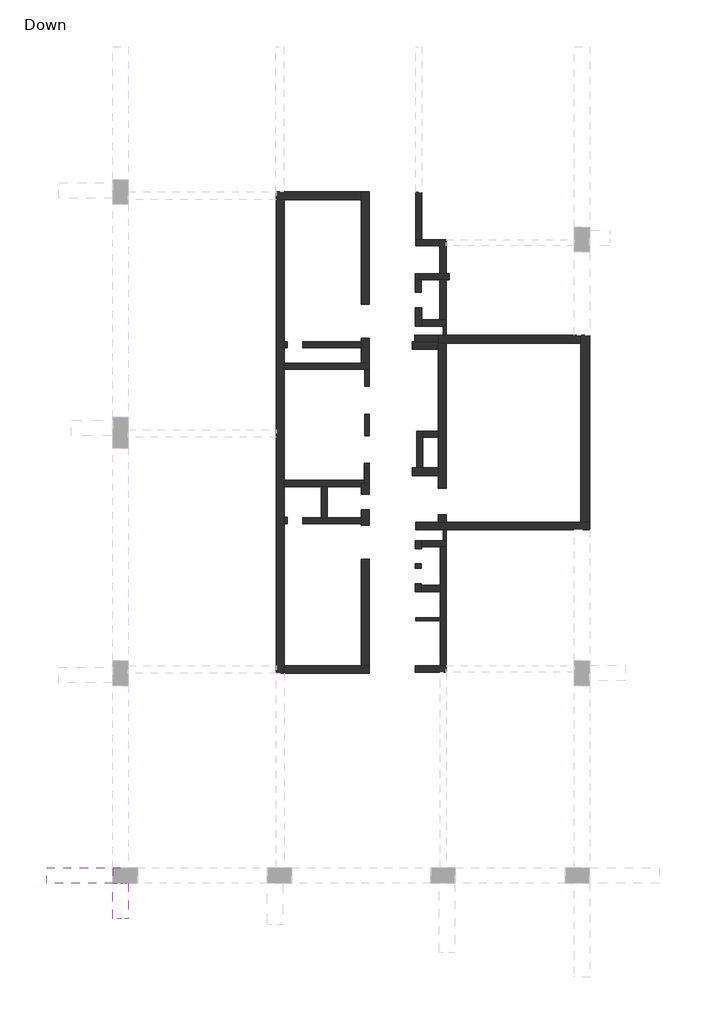
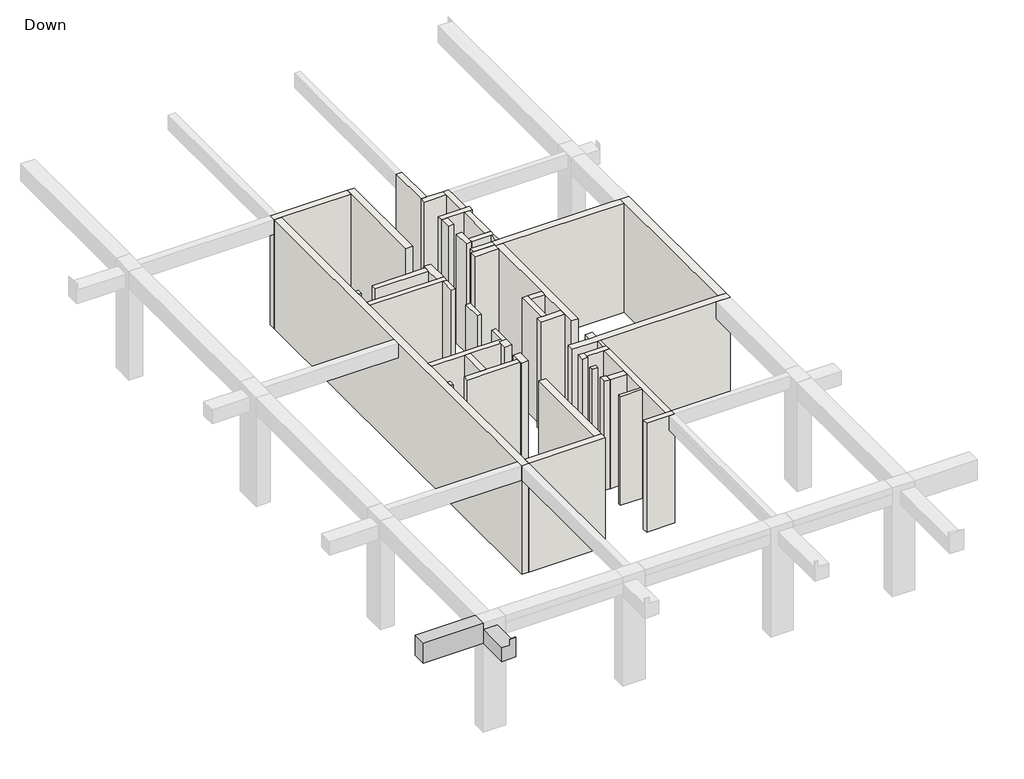
# One storey, part 1 of 2: 46 walls, 2 beams.
"""IFC4 building model written with IfcOpenShell, lengths in millimetres."""

from ifc_helpers import new_model, si_unit, origin, origin_with_axes, place, context, project, spatial, polyline, outline, extrude, faceted_brep, element, save

model = new_model("IFC4")

# Units and contexts
model_context = context("Model", 3, world=origin())
ifc_project = project(units=[si_unit("LENGTHUNIT", "METRE", prefix="MILLI")], contexts=[model_context])

# Site, building, storey
site = spatial("IfcSite", under=ifc_project)
building = spatial("IfcBuilding", under=site)
storey = spatial("IfcBuildingStorey", under=building, Name="Down", Elevation=0.0)

# Beams
placement = place(None, origin())
element("IfcBeam", 1, ObjectType="Concrete Rectengular Beam : 50/75", at=placement, inside=storey, context=model_context, shape_type="Brep", body=[
    faceted_brep([(-11204.7039512, -6829.8142121, 4125.0), (-11204.7039512, -6329.8142121, 4125.0), (-11204.7039512, -6329.8142121, 3375.0), (-11204.7039512, -6829.8142121, 3375.0), (-9054.7039512, -6829.8142121, 4125.0), (-9054.7039512, -6329.9837689, 4125.0), (-9054.7039512, -6329.8142121, 4125.0), (-9054.7039512, -6329.8142121, 3895.0), (-9054.7039512, -6329.8142121, 3475.0), (-8554.7039512, -6329.8142121, 3475.0), (-8554.7039512, -6329.8142121, 3375.0), (-8554.7039512, -6329.9837689, 3375.0), (-9054.7039512, -6329.9837689, 3375.0), (-9054.7039512, -6829.8142121, 3375.0), (-8554.7039512, -6329.9837689, 3475.0), (-9054.7039512, -6329.9837689, 3475.0)], [[[0, 1, 2, 3]], [[1, 0, 4, 5, 6]], [[2, 1, 6, 7, 8, 9, 10]], [[3, 2, 10, 11, 12, 13]], [[0, 3, 13, 4]], [[11, 10, 9, 14]], [[13, 12, 15, 8, 7, 6, 5, 4]], [[12, 11, 14, 15]], [[8, 15, 14, 9]]]),
])
element("IfcBeam", 2, ObjectType="Concrete Rectengular Beam : 50/75", at=placement, inside=storey, context=model_context, shape_type="Brep", body=[
    faceted_brep([(-9054.7039512, -7979.9837689, 3375.0), (-8554.7039512, -7979.9837689, 3375.0), (-8554.7039512, -7979.9837689, 4125.0), (-8777.1634353, -7979.9837689, 4125.0), (-8777.1634353, -7979.9837689, 3895.0), (-9054.7039512, -7979.9837689, 3895.0), (-8554.7039512, -7947.7950382, 4125.0), (-9054.7039512, -6829.9837689, 3375.0), (-9054.7039512, -6829.9837689, 3895.0), (-8554.7039512, -6829.9837689, 3375.0), (-8554.7039512, -6829.9837689, 3475.0), (-8554.7039512, -6829.9837689, 3895.0), (-8554.7039512, -7947.7950382, 3895.0), (-8804.7039512, -6829.9837689, 3895.0), (-8804.7039512, -6829.9837689, 3475.0), (-8655.7238806, -6829.9837689, 3475.0), (-8655.7238806, -6829.9837689, 3895.0), (-8655.7238806, -6832.2071205, 3895.0), (-8804.7039512, -6832.2071205, 3895.0), (-8655.7238806, -6832.2071205, 3475.0), (-8804.7039512, -6832.2071205, 3475.0)], [[[0, 1, 2, 3, 4, 5]], [[3, 2, 6]], [[7, 0, 5, 8]], [[1, 0, 7, 9]], [[2, 1, 9, 10, 11, 12, 6]], [[9, 7, 8, 13, 14, 15, 16, 11, 10]], [[4, 12, 11, 16, 17, 18, 13, 8, 5]], [[12, 4, 3, 6]], [[19, 15, 14, 20]], [[19, 20, 18, 17]], [[15, 19, 17, 16]], [[20, 14, 13, 18]]]),
])

# Walls
element("IfcWall", 3, ObjectType="10", at=placement, inside=storey, context=model_context, shape_type="Brep", body=[
    faceted_brep([(1734.634453, 10911.592205, 0.0), (1734.634453, 11211.8466742, 0.0), (1734.634453, 11211.8466742, 4125.0), (1734.634453, 10911.592205, 4125.0), (1734.634453, 10911.592205, 3895.0), (1634.634453, 10911.592205, 0.0), (1634.634453, 10911.592205, 3895.0), (1634.634453, 10911.592205, 4125.0), (1634.634453, 11211.8466742, 4125.0), (1634.634453, 11211.8466742, 3895.0), (1634.634453, 11211.8466742, 0.0)], [[[0, 1, 2, 3, 4]], [[5, 6, 7, 8, 9, 10]], [[1, 0, 5, 10]], [[3, 2, 8, 7]], [[0, 4, 3, 7, 6, 5]], [[2, 1, 10, 9, 8]]]),
])
element("IfcWall", 4, ObjectType="10", at=placement, inside=storey, context=model_context, shape_type="Brep", body=[
    faceted_brep([(1741.4745301, 4266.6343543, 0.0), (1741.4745301, 4616.7541606, 0.0), (1741.4745301, 4616.7541606, 3895.0), (1741.4745301, 4616.7541606, 4125.0), (1741.4745301, 4266.6343543, 4125.0), (1641.4745301, 4266.6343543, 0.0), (1641.4745301, 4266.6343543, 3895.0), (1641.4745301, 4266.6343543, 4125.0), (1641.4745301, 4616.7541606, 4125.0), (1641.4745301, 4616.7541606, 3895.0), (1641.4745301, 4616.7541606, 0.0)], [[[0, 1, 2, 3, 4]], [[5, 6, 7, 8, 9, 10]], [[1, 0, 5, 10]], [[4, 3, 8, 7]], [[3, 2, 1, 10, 9, 8]], [[0, 4, 7, 6, 5]]]),
])
element("IfcWall", 5, ObjectType="10", at=placement, inside=storey, context=model_context, shape_type="Brep", body=[
    faceted_brep([(1541.4745301, 1765.7881778, 0.0), (754.6005416, 1765.7881778, 0.0), (754.6005416, 1765.7881778, 3895.0), (754.6005416, 1765.7881778, 4125.0), (1541.4745301, 1765.7881778, 4125.0), (1541.4745301, 1765.7881778, 3895.0), (1541.4745301, 1665.7881778, 0.0), (1541.4745301, 1665.7881778, 3895.0), (1541.4745301, 1665.7881778, 4125.0), (754.6005416, 1665.7881778, 4125.0), (754.6005416, 1665.7881778, 3895.0), (754.6005416, 1665.7881778, 0.0)], [[[0, 1, 2, 3, 4, 5]], [[6, 7, 8, 9, 10, 11]], [[1, 0, 6, 11]], [[3, 2, 1, 11, 10, 9]], [[4, 3, 9, 8]], [[0, 5, 4, 8, 7, 6]]]),
])
element("IfcWall", 6, ObjectType="15", at=placement, inside=storey, context=model_context, shape_type="Brep", body=[
    faceted_brep([(-759.1191868, 6117.2962066, 0.0), (-759.1191868, 6767.4827191, 0.0), (-759.1191868, 6767.4827191, 3895.0), (-759.1191868, 6767.4827191, 4125.0), (-759.1191868, 6117.2962066, 4125.0), (-909.1191868, 6117.2962066, 0.0), (-909.1191868, 6117.2962066, 4125.0), (-909.1191868, 6217.2962066, 4125.0), (-909.1191868, 6767.4827191, 4125.0), (-909.1191868, 6767.4827191, 3895.0), (-909.1191868, 6767.4827191, 0.0), (-909.1191868, 6217.2962066, 0.0)], [[[0, 1, 2, 3, 4]], [[5, 6, 7, 8, 9, 10, 11]], [[1, 0, 5, 11, 10]], [[3, 2, 1, 10, 9, 8]], [[4, 3, 8, 7, 6]], [[0, 4, 6, 5]]]),
])
element("IfcWall", 7, ObjectType="15", at=placement, inside=storey, context=model_context, shape_type="Brep", body=[
    faceted_brep([(-909.0341404, 9811.4395145, 0.0), (-909.0341404, 9271.3725849, 0.0), (-909.0341404, 9271.3725849, 4125.0), (-909.0341404, 9811.4395145, 4125.0), (-759.0341404, 9811.4395145, 0.0), (-759.0341404, 9811.4395145, 4125.0), (-759.0341404, 9271.3725849, 4125.0), (-759.0341404, 9271.3725849, 3895.0), (-759.0341404, 9271.3725849, 0.0), (-759.7631009, 9811.4395145, 0.0), (-759.7631009, 9811.4395145, 4125.0)], [[[0, 1, 2, 3]], [[4, 5, 6, 7, 8]], [[1, 0, 9, 4, 8]], [[2, 1, 8, 7, 6]], [[3, 2, 6, 5, 10]], [[0, 3, 10, 5, 4, 9]]]),
])
element("IfcWall", 8, ObjectType="15", at=placement, inside=storey, context=model_context, shape_type="Brep", body=[
    faceted_brep([(-909.0344977, 8360.8800663, 0.0), (-909.0344977, 7660.8800663, 0.0), (-909.0344977, 7660.8800663, 4125.0), (-909.0344977, 8360.8800663, 4125.0), (-909.0344977, 8360.8800663, 3895.0), (-759.0344977, 8360.8800663, 0.0), (-759.0344977, 8360.8800663, 3895.0), (-759.0344977, 8360.8800663, 4125.0), (-759.0344977, 7660.8800663, 4125.0), (-759.0344977, 7660.8800663, 3895.0), (-759.0344977, 7660.8800663, 0.0)], [[[0, 1, 2, 3, 4]], [[5, 6, 7, 8, 9, 10]], [[1, 0, 5, 10]], [[2, 1, 10, 9, 8]], [[3, 2, 8, 7]], [[0, 4, 3, 7, 6, 5]]]),
])
element("IfcWall", 9, ObjectType="20", at=placement, inside=storey, context=model_context, shape_type="Brep", body=[
    faceted_brep([(-1009.0341404, 5009.6760341, 0.0), (-2109.5601686, 5009.6760341, 0.0), (-2309.5601686, 5009.6760341, 0.0), (-2909.1188742, 5009.6760341, 0.0), (-2909.1188742, 5009.6760341, 4125.0), (-2309.5601686, 5009.6760341, 4125.0), (-2109.5601686, 5009.6760341, 4125.0), (-1009.0341404, 5009.6760341, 4125.0), (-1009.0341404, 4809.6760341, 0.0), (-1009.0341404, 4809.6760341, 4125.0), (-2909.1188742, 4809.6760341, 4125.0), (-2909.1188742, 4809.6760341, 0.0)], [[[0, 1, 2, 3, 4, 5, 6, 7]], [[8, 9, 10, 11]], [[3, 2, 1, 0, 8, 11]], [[4, 3, 11, 10]], [[7, 6, 5, 4, 10, 9]], [[0, 7, 9, 8]]]),
])
element("IfcWall", 10, ObjectType="20", at=placement, inside=storey, context=model_context, shape_type="SweptSolid", body=[
    extrude(outline(polyline([(-3510.0513475, 5016.8224745), (-3409.9328364, 5016.8224745), (-3409.9328364, 4816.8224745), (-3510.0513475, 4816.8224745), (-3510.0513475, 5016.8224745)])), origin_with_axes(), (0.0, 0.0, 1.0), 4125.0),
])
element("IfcWall", 11, ObjectType="20", at=placement, inside=storey, context=model_context, shape_type="Brep", body=[
    faceted_brep([(-909.1191868, 6217.2962066, 0.0), (-3510.0513475, 6217.2962066, 0.0), (-3510.0513475, 6217.2962066, 4125.0), (-909.1191868, 6217.2962066, 4125.0), (-1009.1191868, 6017.2962066, 0.0), (-1009.1191868, 6017.2962066, 4125.0), (-2109.5601686, 6017.2962066, 4125.0), (-2309.5601686, 6017.2962066, 4125.0), (-3510.0513475, 6017.2962066, 4125.0), (-3510.0513475, 6017.2962066, 0.0), (-2309.5601686, 6017.2962066, 0.0), (-2109.5601686, 6017.2962066, 0.0), (-909.1191868, 6117.2962066, 0.0), (-1009.1191868, 6117.2962066, 0.0), (-1009.1191868, 6117.2962066, 4125.0), (-909.1191868, 6117.2962066, 4125.0)], [[[0, 1, 2, 3]], [[4, 5, 6, 7, 8, 9, 10, 11]], [[1, 0, 12, 13, 4, 11, 10, 9]], [[3, 2, 8, 7, 6, 5, 14, 15]], [[0, 3, 15, 12]], [[15, 14, 13, 12]], [[14, 5, 4, 13]], [[2, 1, 9, 8]]]),
])
element("IfcWall", 12, ObjectType="20", at=placement, inside=storey, context=model_context, shape_type="SweptSolid", body=[
    extrude(outline(polyline([(-2309.5601686, 5009.6760341), (-2309.5601686, 6017.2962066), (-2109.5601686, 6017.2962066), (-2109.5601686, 5009.6760341), (-2309.5601686, 5009.6760341)])), origin_with_axes(), (0.0, 0.0, 1.0), 4125.0),
])
element("IfcWall", 13, ObjectType="20", at=placement, inside=storey, context=model_context, shape_type="Brep", body=[
    faceted_brep([(1484.6681857, 10911.592205, 0.0), (724.6681857, 10911.592205, 0.0), (724.6681857, 10911.592205, 3895.0), (724.6681857, 10911.592205, 4125.0), (1484.6681857, 10911.592205, 4125.0), (1484.6681857, 10711.592205, 0.0), (1484.6681857, 10711.592205, 4125.0), (724.6681857, 10711.592205, 4125.0), (724.6681857, 10711.592205, 3895.0), (724.6681857, 10711.592205, 0.0)], [[[0, 1, 2, 3, 4]], [[5, 6, 7, 8, 9]], [[1, 0, 5, 9]], [[3, 2, 1, 9, 8, 7]], [[4, 3, 7, 6]], [[0, 4, 6, 5]]]),
])
element("IfcWall", 14, ObjectType="20", at=placement, inside=storey, context=model_context, shape_type="Brep", body=[
    faceted_brep([(741.4739495, 11812.0494279, 0.0), (741.4739495, 11211.8466742, 0.0), (741.4739495, 11211.8466742, 3895.0), (741.4739495, 11211.8466742, 4125.0), (741.4739495, 11812.0494279, 4125.0), (741.4739495, 11812.0494279, 3895.0), (941.4739495, 11812.0494279, 0.0), (941.4739495, 11812.0494279, 3895.0), (941.4739495, 11812.0494279, 4125.0), (941.4739495, 11411.8466742, 4125.0), (941.4739495, 11211.8466742, 4125.0), (941.4739495, 11211.8466742, 0.0), (941.4739495, 11411.8466742, 0.0)], [[[0, 1, 2, 3, 4, 5]], [[6, 7, 8, 9, 10, 11, 12]], [[1, 0, 6, 12, 11]], [[4, 3, 10, 9, 8]], [[0, 5, 4, 8, 7, 6]], [[3, 2, 1, 11, 10]]]),
])
element("IfcWall", 15, ObjectType="20", at=placement, inside=storey, context=model_context, shape_type="Brep", body=[
    faceted_brep([(941.4739495, 11211.8466742, 0.0), (1634.634453, 11211.8466742, 0.0), (1734.6683644, 11211.8466742, 0.0), (1734.6683644, 11211.8466742, 4125.0), (1634.634453, 11211.8466742, 4125.0), (941.4739495, 11211.8466742, 4125.0), (941.4739495, 11411.8466742, 0.0), (941.4739495, 11411.8466742, 3895.0), (941.4739495, 11411.8466742, 4125.0), (1534.6683644, 11411.8466742, 4125.0), (1734.6683644, 11411.8466742, 4125.0), (1734.6683644, 11411.8466742, 0.0), (1534.6683644, 11411.8466742, 0.0)], [[[0, 1, 2, 3, 4, 5]], [[6, 7, 8, 9, 10, 11, 12]], [[2, 1, 0, 6, 12, 11]], [[5, 4, 3, 10, 9, 8]], [[0, 5, 8, 7, 6]], [[3, 2, 11, 10]]]),
])
element("IfcWall", 16, ObjectType="20", at=placement, inside=storey, context=model_context, shape_type="Brep", body=[
    faceted_brep([(1734.6683644, 11411.8466742, 0.0), (1734.6683644, 12711.8466742, 0.0), (1734.6683644, 12711.8466742, 3895.0), (1734.6683644, 12711.8466742, 4125.0), (1734.6683644, 11411.8466742, 4125.0), (1534.6683644, 11411.8466742, 0.0), (1534.6683644, 11411.8466742, 3895.0), (1534.6683644, 11411.8466742, 4125.0), (1534.6683644, 12711.8466742, 4125.0), (1534.6683644, 12711.8466742, 3895.0), (1534.6683644, 12711.8466742, 0.0)], [[[0, 1, 2, 3, 4]], [[5, 6, 7, 8, 9, 10]], [[1, 0, 5, 10]], [[4, 3, 8, 7]], [[0, 4, 7, 6, 5]], [[3, 2, 1, 10, 9, 8]]]),
])
element("IfcWall", 17, ObjectType="20", at=placement, inside=storey, context=model_context, shape_type="Brep", body=[
    faceted_brep([(1834.7023204, 12911.8466742, 0.0), (1734.6005416, 12911.8466742, 0.0), (1534.6005416, 12911.8466742, 0.0), (734.6683644, 12911.8466742, 0.0), (734.6683644, 12911.8466742, 3895.0), (734.6683644, 12911.8466742, 4125.0), (1534.6005416, 12911.8466742, 4125.0), (1734.6005416, 12911.8466742, 4125.0), (1834.7023204, 12911.8466742, 4125.0), (1834.7023204, 12911.8466742, 3895.0), (1834.7023204, 12711.8466742, 0.0), (1834.7023204, 12711.8466742, 3895.0), (1834.7023204, 12711.8466742, 4125.0), (1734.6683644, 12711.8466742, 4125.0), (1534.6683644, 12711.8466742, 4125.0), (934.6683644, 12711.8466742, 4125.0), (734.6683644, 12711.8466742, 4125.0), (734.6683644, 12711.8466742, 0.0), (934.6683644, 12711.8466742, 0.0), (1534.6683644, 12711.8466742, 0.0), (1734.6683644, 12711.8466742, 0.0)], [[[0, 1, 2, 3, 4, 5, 6, 7, 8, 9]], [[10, 11, 12, 13, 14, 15, 16, 17, 18, 19, 20]], [[3, 2, 1, 0, 10, 20, 19, 18, 17]], [[8, 7, 6, 5, 16, 15, 14, 13, 12]], [[0, 9, 8, 12, 11, 10]], [[5, 4, 3, 17, 16]]]),
])
element("IfcWall", 18, ObjectType="20", at=placement, inside=storey, context=model_context, shape_type="Brep", body=[
    faceted_brep([(734.6683644, 12711.8466742, 0.0), (734.6683644, 12311.8466742, 0.0), (734.6683644, 12311.8466742, 3895.0), (734.6683644, 12311.8466742, 4125.0), (734.6683644, 12711.8466742, 4125.0), (934.6683644, 12711.8466742, 0.0), (934.6683644, 12711.8466742, 3895.0), (934.6683644, 12711.8466742, 4125.0), (934.6683644, 12311.8466742, 4125.0), (934.6683644, 12311.8466742, 3895.0), (934.6683644, 12311.8466742, 0.0)], [[[0, 1, 2, 3, 4]], [[5, 6, 7, 8, 9, 10]], [[1, 0, 5, 10]], [[3, 2, 1, 10, 9, 8]], [[4, 3, 8, 7]], [[0, 4, 7, 6, 5]]]),
])
element("IfcWall", 19, ObjectType="20", at=placement, inside=storey, context=model_context, shape_type="Brep", body=[
    faceted_brep([(1734.6005416, 12911.8466742, 0.0), (1734.6005416, 14012.7962372, 0.0), (1734.6005416, 14012.7962372, 4125.0), (1734.6005416, 13812.7962372, 4125.0), (1734.6005416, 12911.8466742, 4125.0), (1734.6005416, 12911.8466742, 3895.0), (1534.6005416, 12911.8466742, 0.0), (1534.6005416, 12911.8466742, 3895.0), (1534.6005416, 12911.8466742, 4125.0), (1534.6005416, 13812.7962372, 4125.0), (1534.6005416, 14012.7962372, 4125.0), (1534.6005416, 14012.7962372, 0.0), (1534.6005416, 13812.7962372, 0.0)], [[[0, 1, 2, 3, 4, 5]], [[6, 7, 8, 9, 10, 11, 12]], [[1, 0, 6, 12, 11]], [[4, 3, 2, 10, 9, 8]], [[2, 1, 11, 10]], [[0, 5, 4, 8, 7, 6]]]),
])
element("IfcWall", 20, ObjectType="20", at=placement, inside=storey, context=model_context, shape_type="Brep", body=[
    faceted_brep([(1534.6005416, 14012.7962372, 0.0), (945.9739967, 14012.7962372, 0.0), (745.9739967, 14012.7962372, 0.0), (745.9739967, 14012.7962372, 4125.0), (945.9739967, 14012.7962372, 4125.0), (1534.6005416, 14012.7962372, 4125.0), (1534.6005416, 13812.7962372, 0.0), (1534.6005416, 13812.7962372, 3895.0), (1534.6005416, 13812.7962372, 4125.0), (745.9739967, 13812.7962372, 4125.0), (745.9739967, 13812.7962372, 3895.0), (745.9739967, 13812.7962372, 0.0)], [[[0, 1, 2, 3, 4, 5]], [[6, 7, 8, 9, 10, 11]], [[2, 1, 0, 6, 11]], [[5, 4, 3, 9, 8]], [[0, 5, 8, 7, 6]], [[3, 2, 11, 10, 9]]]),
])
element("IfcWall", 21, ObjectType="20", at=placement, inside=storey, context=model_context, shape_type="Brep", body=[
    faceted_brep([(945.9739967, 14012.7962372, 0.0), (945.9739967, 15552.7962372, 0.0), (945.9739967, 15552.7962372, 3575.0), (945.9739967, 15552.7962372, 4125.0), (945.9739967, 14012.7962372, 4125.0), (945.9739967, 14012.7962372, 3895.0), (745.9739967, 14012.7962372, 0.0), (745.9739967, 14012.7962372, 4125.0), (745.9739967, 15552.7962372, 4125.0), (745.9739967, 15552.7962372, 3575.0), (745.9739967, 15552.7962372, 0.0)], [[[0, 1, 2, 3, 4, 5]], [[6, 7, 8, 9, 10]], [[1, 0, 6, 10]], [[3, 2, 1, 10, 9, 8]], [[4, 3, 8, 7]], [[0, 5, 4, 7, 6]]]),
])
element("IfcWall", 22, ObjectType="20", at=placement, inside=storey, context=model_context, shape_type="SweptSolid", body=[
    extrude(outline(polyline([(-1009.7631009, 10511.6779659), (-2909.7631009, 10511.6779659), (-2909.7631009, 10711.6779659), (-1009.7631009, 10711.6779659), (-1009.7631009, 10511.6779659)])), origin_with_axes(), (0.0, 0.0, 1.0), 4125.0),
])
element("IfcWall", 23, ObjectType="20", at=placement, inside=storey, context=model_context, shape_type="SweptSolid", body=[
    extrude(outline(polyline([(-3510.0513475, 10711.6772513), (-3409.9328364, 10711.6772513), (-3409.9328364, 10511.6772513), (-3510.0513475, 10511.6772513), (-3510.0513475, 10711.6772513)])), origin_with_axes(), (0.0, 0.0, 1.0), 4125.0),
])
element("IfcWall", 24, ObjectType="20", at=placement, inside=storey, context=model_context, shape_type="Brep", body=[
    faceted_brep([(-759.7631009, 10011.4395145, 0.0), (-1009.7631009, 10011.4395145, 0.0), (-3510.0513475, 10011.4395145, 0.0), (-3510.0513475, 10011.4395145, 4125.0), (-1009.7631009, 10011.4395145, 4125.0), (-759.7631009, 10011.4395145, 4125.0), (-759.7631009, 9811.4395145, 0.0), (-759.7631009, 9811.4395145, 4125.0), (-909.0341404, 9811.4395145, 4125.0), (-3510.0513475, 9811.4395145, 4125.0), (-3510.0513475, 9811.4395145, 0.0), (-909.0341404, 9811.4395145, 0.0)], [[[0, 1, 2, 3, 4, 5]], [[6, 7, 8, 9, 10, 11]], [[2, 1, 0, 6, 11, 10]], [[5, 4, 3, 9, 8, 7]], [[3, 2, 10, 9]], [[0, 5, 7, 6]]]),
])
element("IfcWall", 25, ObjectType="20", at=placement, inside=storey, context=model_context, shape_type="Brep", body=[
    faceted_brep([(984.3467423, 6617.3474309, 0.0), (984.3467423, 7610.6935537, 0.0), (984.3467423, 7810.6935537, 0.0), (984.3467423, 7810.6935537, 4125.0), (984.3467423, 7610.6935537, 4125.0), (984.3467423, 6617.3474309, 4125.0), (784.3467423, 6617.3474309, 0.0), (784.3467423, 6617.3474309, 3895.0), (784.3467423, 6617.3474309, 4125.0), (784.3467423, 7810.6935537, 4125.0), (784.3467423, 7810.6935537, 3895.0), (784.3467423, 7810.6935537, 0.0)], [[[0, 1, 2, 3, 4, 5]], [[6, 7, 8, 9, 10, 11]], [[2, 1, 0, 6, 11]], [[5, 4, 3, 9, 8]], [[0, 5, 8, 7, 6]], [[3, 2, 11, 10, 9]]]),
])
element("IfcWall", 26, ObjectType="20", at=placement, inside=storey, context=model_context, shape_type="Brep", body=[
    faceted_brep([(984.3467423, 7610.6935537, 0.0), (1484.6681857, 7610.6935537, 0.0), (1484.6681857, 7610.6935537, 4125.0), (984.3467423, 7610.6935537, 4125.0), (984.3467423, 7810.6935537, 0.0), (984.3467423, 7810.6935537, 4125.0), (1484.6681857, 7810.6935537, 4125.0), (1484.6681857, 7810.6935537, 3895.0), (1484.6681857, 7810.6935537, 0.0)], [[[0, 1, 2, 3]], [[4, 5, 6, 7, 8]], [[1, 0, 4, 8]], [[3, 2, 6, 5]], [[0, 3, 5, 4]], [[2, 1, 8, 7, 6]]]),
])
element("IfcWall", 27, ObjectType="20", at=placement, inside=storey, context=model_context, shape_type="Brep", body=[
    faceted_brep([(941.4745301, 4066.6343543, 0.0), (1541.4745301, 4066.6343543, 0.0), (1741.4745301, 4066.6343543, 0.0), (1741.4745301, 4066.6343543, 4125.0), (1541.4745301, 4066.6343543, 4125.0), (941.4745301, 4066.6343543, 4125.0), (941.4745301, 4066.6343543, 3895.0), (941.4745301, 4266.6343543, 0.0), (941.4745301, 4266.6343543, 4125.0), (1641.4745301, 4266.6343543, 4125.0), (1741.4745301, 4266.6343543, 4125.0), (1741.4745301, 4266.6343543, 0.0), (1641.4745301, 4266.6343543, 0.0)], [[[0, 1, 2, 3, 4, 5, 6]], [[7, 8, 9, 10, 11, 12]], [[2, 1, 0, 7, 12, 11]], [[5, 4, 3, 10, 9, 8]], [[3, 2, 11, 10]], [[0, 6, 5, 8, 7]]]),
])
element("IfcWall", 28, ObjectType="20", at=placement, inside=storey, context=model_context, shape_type="Brep", body=[
    faceted_brep([(741.4745301, 4266.6343543, 0.0), (741.4745301, 4006.6343543, 0.0), (741.4745301, 4006.6343543, 3895.0), (741.4745301, 4006.6343543, 4125.0), (741.4745301, 4266.6343543, 4125.0), (741.4745301, 4266.6343543, 3895.0), (941.4745301, 4266.6343543, 0.0), (941.4745301, 4266.6343543, 4125.0), (941.4745301, 4066.6343543, 4125.0), (941.4745301, 4006.6343543, 4125.0), (941.4745301, 4006.6343543, 3895.0), (941.4745301, 4006.6343543, 0.0), (941.4745301, 4066.6343543, 0.0)], [[[0, 1, 2, 3, 4, 5]], [[6, 7, 8, 9, 10, 11, 12]], [[1, 0, 6, 12, 11]], [[3, 2, 1, 11, 10, 9]], [[4, 3, 9, 8, 7]], [[0, 5, 4, 7, 6]]]),
])
element("IfcWall", 29, ObjectType="20", at=placement, inside=storey, context=model_context, shape_type="Brep", body=[
    faceted_brep([(734.3288041, 3516.3799744, 0.0), (734.3288041, 3366.3290627, 0.0), (734.3288041, 3366.3290627, 3895.0), (734.3288041, 3366.3290627, 4125.0), (734.3288041, 3516.3799744, 4125.0), (734.3288041, 3516.3799744, 3895.0), (934.3288041, 3516.3799744, 0.0), (934.3288041, 3516.3799744, 3895.0), (934.3288041, 3516.3799744, 4125.0), (934.3288041, 3366.3290627, 4125.0), (934.3288041, 3366.3290627, 3895.0), (934.3288041, 3366.3290627, 0.0)], [[[0, 1, 2, 3, 4, 5]], [[6, 7, 8, 9, 10, 11]], [[1, 0, 6, 11]], [[3, 2, 1, 11, 10, 9]], [[4, 3, 9, 8]], [[0, 5, 4, 8, 7, 6]]]),
])
element("IfcWall", 30, ObjectType="20", at=placement, inside=storey, context=model_context, shape_type="Brep", body=[
    faceted_brep([(734.3288041, 2866.1594612, 0.0), (734.3288041, 2616.6343543, 0.0), (734.3288041, 2616.6343543, 3895.0), (734.3288041, 2616.6343543, 4125.0), (734.3288041, 2866.1594612, 4125.0), (734.3288041, 2866.1594612, 3895.0), (934.3288041, 2866.1594612, 0.0), (934.3288041, 2866.1594612, 3895.0), (934.3288041, 2866.1594612, 4125.0), (934.3288041, 2816.6343543, 4125.0), (934.3288041, 2616.6343543, 4125.0), (934.3288041, 2616.6343543, 0.0), (934.3288041, 2816.6343543, 0.0)], [[[0, 1, 2, 3, 4, 5]], [[6, 7, 8, 9, 10, 11, 12]], [[1, 0, 6, 12, 11]], [[4, 3, 10, 9, 8]], [[0, 5, 4, 8, 7, 6]], [[3, 2, 1, 11, 10]]]),
])
element("IfcWall", 31, ObjectType="20", at=placement, inside=storey, context=model_context, shape_type="Brep", body=[
    faceted_brep([(934.3288041, 2616.6343543, 0.0), (1541.4745301, 2616.6343543, 0.0), (1541.4745301, 2616.6343543, 3895.0), (1541.4745301, 2616.6343543, 4125.0), (934.3288041, 2616.6343543, 4125.0), (934.3288041, 2816.6343543, 0.0), (934.3288041, 2816.6343543, 3895.0), (934.3288041, 2816.6343543, 4125.0), (1541.4745301, 2816.6343543, 4125.0), (1541.4745301, 2816.6343543, 3895.0), (1541.4745301, 2816.6343543, 0.0)], [[[0, 1, 2, 3, 4]], [[5, 6, 7, 8, 9, 10]], [[1, 0, 5, 10]], [[4, 3, 8, 7]], [[0, 4, 7, 6, 5]], [[3, 2, 1, 10, 9, 8]]]),
])
element("IfcWall", 32, ObjectType="20", at=placement, inside=storey, context=model_context, shape_type="Brep", body=[
    faceted_brep([(1541.4745301, 4066.6343543, 0.0), (1541.4745301, 2816.6343543, 0.0), (1541.4745301, 2616.6343543, 0.0), (1541.4745301, 1765.7881778, 0.0), (1541.4745301, 1665.7881778, 0.0), (1541.4745301, 206.0759332, 0.0), (1541.4745301, 206.0759332, 3895.0), (1541.4745301, 206.0759332, 4125.0), (1541.4745301, 1665.7881778, 4125.0), (1541.4745301, 1765.7881778, 4125.0), (1541.4745301, 2616.6343543, 4125.0), (1541.4745301, 2816.6343543, 4125.0), (1541.4745301, 4066.6343543, 4125.0), (1541.4745301, 4066.6343543, 3895.0), (1741.4745301, 4066.6343543, 0.0), (1741.4745301, 4066.6343543, 4125.0), (1741.4745301, 206.0759332, 4125.0), (1741.4745301, 206.0759332, 3895.0), (1741.4745301, 206.0759332, 0.0)], [[[0, 1, 2, 3, 4, 5, 6, 7, 8, 9, 10, 11, 12, 13]], [[14, 15, 16, 17, 18]], [[5, 4, 3, 2, 1, 0, 14, 18]], [[12, 11, 10, 9, 8, 7, 16, 15]], [[0, 13, 12, 15, 14]], [[7, 6, 5, 18, 17, 16]]]),
])
element("IfcWall", 33, ObjectType="20", at=placement, inside=storey, context=model_context, shape_type="Brep", body=[
    faceted_brep([(1741.4745301, 206.0759332, 0.0), (1541.4745301, 206.0759332, 0.0), (737.8283053, 206.0759332, 0.0), (737.8283053, 206.0759332, 4125.0), (1541.4745301, 206.0759332, 4125.0), (1741.4745301, 206.0759332, 4125.0), (1741.4745301, 206.0759332, 3625.0), (1741.4745301, 6.0759332, 0.0), (1741.4745301, 6.0759332, 3575.0), (1741.4745301, 6.0759332, 3625.0), (1741.4745301, 6.0759332, 4125.0), (1541.8129739, 6.0759332, 4125.0), (737.8283053, 6.0759332, 4125.0), (737.8283053, 6.0759332, 0.0)], [[[0, 1, 2, 3, 4, 5, 6]], [[7, 8, 9, 10, 11, 12, 13]], [[2, 1, 0, 7, 13]], [[3, 2, 13, 12]], [[5, 4, 3, 12, 11, 10]], [[0, 6, 5, 10, 9, 8, 7]]]),
])
element("IfcWall", 34, ObjectType="25", at=placement, inside=storey, context=model_context, shape_type="Brep", body=[
    faceted_brep([(744.5830054, 4616.7541606, 0.0), (1641.4745301, 4616.7541606, 0.0), (1741.4745301, 4616.7541606, 0.0), (6386.2445731, 4616.7541606, 0.0), (6386.2445731, 4616.7541606, 3895.0), (6386.2445731, 4616.7541606, 4125.0), (5886.2445731, 4616.7541606, 4125.0), (1741.4745301, 4616.7541606, 4125.0), (1641.4745301, 4616.7541606, 4125.0), (744.5830054, 4616.7541606, 4125.0), (744.5830054, 4616.7541606, 3895.0), (744.5830054, 4866.7541606, 0.0), (744.5830054, 4866.7541606, 3895.0), (744.5830054, 4866.7541606, 4125.0), (1484.5830054, 4866.7541606, 4125.0), (1734.5830054, 4866.7541606, 4125.0), (6086.2445731, 4866.7541606, 4125.0), (6386.2445731, 4866.7541606, 4125.0), (6386.2445731, 4866.7541606, 0.0), (6086.2445731, 4866.7541606, 0.0), (1734.5830054, 4866.7541606, 0.0), (1484.5830054, 4866.7541606, 0.0)], [[[0, 1, 2, 3, 4, 5, 6, 7, 8, 9, 10]], [[11, 12, 13, 14, 15, 16, 17, 18, 19, 20, 21]], [[3, 2, 1, 0, 11, 21, 20, 19, 18]], [[9, 8, 7, 6, 5, 17, 16, 15, 14, 13]], [[0, 10, 9, 13, 12, 11]], [[5, 4, 3, 18, 17]]]),
])
element("IfcWall", 35, ObjectType="25", at=placement, inside=storey, context=model_context, shape_type="Brep", body=[
    faceted_brep([(6086.2445731, 10911.592205, 0.0), (1734.634453, 10911.592205, 0.0), (1634.634453, 10911.592205, 0.0), (1484.6681857, 10911.592205, 0.0), (1484.6681857, 10911.592205, 4125.0), (1634.634453, 10911.592205, 4125.0), (1734.634453, 10911.592205, 4125.0), (5886.2445731, 10911.592205, 4125.0), (6086.2445731, 10911.592205, 4125.0), (6086.2445731, 10661.592205, 0.0), (6086.2445731, 10661.592205, 3895.0), (6086.2445731, 10661.592205, 4125.0), (1734.6681857, 10661.592205, 4125.0), (1484.6681857, 10661.592205, 4125.0), (1484.6681857, 10661.592205, 0.0), (1734.6681857, 10661.592205, 0.0), (1484.6681857, 10711.592205, 0.0), (1484.6681857, 10711.592205, 4125.0)], [[[0, 1, 2, 3, 4, 5, 6, 7, 8]], [[9, 10, 11, 12, 13, 14, 15]], [[3, 2, 1, 0, 9, 15, 14, 16]], [[8, 7, 6, 5, 4, 17, 13, 12, 11]], [[0, 8, 11, 10, 9]], [[4, 3, 16, 14, 13, 17]]]),
])
element("IfcWall", 36, ObjectType="25", at=placement, inside=storey, context=model_context, shape_type="Brep", body=[
    faceted_brep([(-759.1188742, 11912.0840984, 0.0), (-759.1188742, 15556.1764947, 0.0), (-759.1188742, 15556.1764947, 3895.0), (-759.1188742, 15556.1764947, 4125.0), (-759.1188742, 11912.0840984, 4125.0), (-759.1188742, 11912.0840984, 3895.0), (-1009.1188742, 11912.0840984, 0.0), (-1009.1188742, 11912.0840984, 4125.0), (-1009.1188742, 15306.1764947, 4125.0), (-1009.1188742, 15556.1764947, 4125.0), (-1009.1188742, 15556.1764947, 0.0), (-1009.1188742, 15306.1764947, 0.0)], [[[0, 1, 2, 3, 4, 5]], [[6, 7, 8, 9, 10, 11]], [[1, 0, 6, 11, 10]], [[4, 3, 9, 8, 7]], [[0, 5, 4, 7, 6]], [[3, 2, 1, 10, 9]]]),
])
element("IfcWall", 37, ObjectType="25", at=placement, inside=storey, context=model_context, shape_type="Brep", body=[
    faceted_brep([(-1009.1188742, 15556.1764947, 0.0), (-3760.0513475, 15556.1764947, 0.0), (-3760.0513475, 15556.1764947, 3575.0), (-3760.0513475, 15556.1764947, 4125.0), (-3529.0260033, 15556.1764947, 4125.0), (-1009.1188742, 15556.1764947, 4125.0), (-1009.1188742, 15306.1764947, 0.0), (-1009.1188742, 15306.1764947, 4125.0), (-3510.0513475, 15306.1764947, 4125.0), (-3760.0513475, 15306.1764947, 4125.0), (-3760.0513475, 15306.1764947, 3575.0), (-3760.0513475, 15306.1764947, 0.0), (-3510.0513475, 15306.1764947, 0.0)], [[[0, 1, 2, 3, 4, 5]], [[6, 7, 8, 9, 10, 11, 12]], [[1, 0, 6, 12, 11]], [[5, 4, 3, 9, 8, 7]], [[0, 5, 7, 6]], [[3, 2, 1, 11, 10, 9]]]),
])
element("IfcWall", 38, ObjectType="25", at=placement, inside=storey, context=model_context, shape_type="Brep", body=[
    faceted_brep([(-3760.0513475, 15306.1764947, 0.0), (-3760.0513475, -34.8235665, 0.0), (-3760.0513475, -34.8235665, 3575.0), (-3760.0513475, -34.8235665, 4125.0), (-3760.0513475, 215.1764335, 4125.0), (-3760.0513475, 7610.6259096, 4125.0), (-3760.0513475, 7860.6259096, 4125.0), (-3760.0513475, 15306.1764947, 4125.0), (-3760.0513475, 15306.1764947, 3895.0), (-3510.0513475, 15306.1764947, 0.0), (-3510.0513475, 15306.1764947, 4125.0), (-3510.0513475, 10711.6772513, 4125.0), (-3510.0513475, 10511.6772513, 4125.0), (-3510.0513475, 10011.4395145, 4125.0), (-3510.0513475, 9811.4395145, 4125.0), (-3510.0513475, 6217.2962066, 4125.0), (-3510.0513475, 6017.2962066, 4125.0), (-3510.0513475, 5016.8224745, 4125.0), (-3510.0513475, 4816.8224745, 4125.0), (-3510.0513475, 215.1764335, 4125.0), (-3510.0513475, -34.8235665, 4125.0), (-3510.0513475, -34.8235665, 3575.0), (-3510.0513475, -34.8235665, 0.0), (-3510.0513475, 215.1764335, 0.0), (-3510.0513475, 4816.8224745, 0.0), (-3510.0513475, 5016.8224745, 0.0), (-3510.0513475, 6017.2962066, 0.0), (-3510.0513475, 6217.2962066, 0.0), (-3510.0513475, 9811.4395145, 0.0), (-3510.0513475, 10011.4395145, 0.0), (-3510.0513475, 10511.6772513, 0.0), (-3510.0513475, 10711.6772513, 0.0)], [[[0, 1, 2, 3, 4, 5, 6, 7, 8]], [[9, 10, 11, 12, 13, 14, 15, 16, 17, 18, 19, 20, 21, 22, 23, 24, 25, 26, 27, 28, 29, 30, 31]], [[1, 0, 9, 31, 30, 29, 28, 27, 26, 25, 24, 23, 22]], [[7, 6, 5, 4, 3, 20, 19, 18, 17, 16, 15, 14, 13, 12, 11, 10]], [[0, 8, 7, 10, 9]], [[3, 2, 1, 22, 21, 20]]]),
])
element("IfcWall", 39, ObjectType="25", at=placement, inside=storey, context=model_context, shape_type="Brep", body=[
    faceted_brep([(-3510.0513475, -34.8235665, 0.0), (-760.0513475, -34.8235665, 0.0), (-760.0513475, -34.8235665, 3895.0), (-760.0513475, -34.8235665, 4125.0), (-3510.0513475, -34.8235665, 4125.0), (-3510.0513475, -34.8235665, 3895.0), (-3510.0513475, 215.1764335, 0.0), (-3510.0513475, 215.1764335, 4125.0), (-1010.0513475, 215.1764335, 4125.0), (-760.0513475, 215.1764335, 4125.0), (-760.0513475, 215.1764335, 0.0), (-1010.0513475, 215.1764335, 0.0)], [[[0, 1, 2, 3, 4, 5]], [[6, 7, 8, 9, 10, 11]], [[1, 0, 6, 11, 10]], [[4, 3, 9, 8, 7]], [[0, 5, 4, 7, 6]], [[3, 2, 1, 10, 9]]]),
])
element("IfcWall", 40, ObjectType="25", at=placement, inside=storey, context=model_context, shape_type="Brep", body=[
    faceted_brep([(-760.0513475, 215.1764335, 0.0), (-760.0513475, 3665.1764335, 0.0), (-760.0513475, 3665.1764335, 3895.0), (-760.0513475, 3665.1764335, 4125.0), (-760.0513475, 215.1764335, 4125.0), (-1010.0513475, 215.1764335, 0.0), (-1010.0513475, 215.1764335, 4125.0), (-1010.0513475, 3665.1764335, 4125.0), (-1010.0513475, 3665.1764335, 3895.0), (-1010.0513475, 3665.1764335, 0.0)], [[[0, 1, 2, 3, 4]], [[5, 6, 7, 8, 9]], [[1, 0, 5, 9]], [[3, 2, 1, 9, 8, 7]], [[4, 3, 7, 6]], [[0, 4, 6, 5]]]),
])
element("IfcWall", 41, ObjectType="25", at=placement, inside=storey, context=model_context, shape_type="Brep", body=[
    faceted_brep([(-1009.0341404, 5266.9740486, 0.0), (-1009.0341404, 5009.6760341, 0.0), (-1009.0341404, 4809.6760341, 0.0), (-1009.0341404, 4766.8045364, 0.0), (-1009.0341404, 4766.8045364, 4125.0), (-1009.0341404, 4809.6760341, 4125.0), (-1009.0341404, 5009.6760341, 4125.0), (-1009.0341404, 5266.9740486, 4125.0), (-1009.0341404, 5266.9740486, 3895.0), (-759.0341404, 5266.9740486, 0.0), (-759.0341404, 5266.9740486, 3895.0), (-759.0341404, 5266.9740486, 4125.0), (-759.0341404, 4766.8045364, 4125.0), (-759.0341404, 4766.8045364, 3895.0), (-759.0341404, 4766.8045364, 0.0)], [[[0, 1, 2, 3, 4, 5, 6, 7, 8]], [[9, 10, 11, 12, 13, 14]], [[3, 2, 1, 0, 9, 14]], [[4, 3, 14, 13, 12]], [[7, 6, 5, 4, 12, 11]], [[0, 8, 7, 11, 10, 9]]]),
])
element("IfcWall", 42, ObjectType="25", at=placement, inside=storey, context=model_context, shape_type="Brep", body=[
    faceted_brep([(-759.1191868, 5767.1435608, 0.0), (-759.1191868, 6117.2962066, 0.0), (-759.1191868, 6117.2962066, 4125.0), (-759.1191868, 5767.1435608, 4125.0), (-759.1191868, 5767.1435608, 3895.0), (-1009.1191868, 5767.1435608, 0.0), (-1009.1191868, 5767.1435608, 4125.0), (-1009.1191868, 6017.2962066, 4125.0), (-1009.1191868, 6117.2962066, 4125.0), (-1009.1191868, 6117.2962066, 0.0), (-1009.1191868, 6017.2962066, 0.0), (-909.1191868, 6117.2962066, 0.0), (-909.1191868, 6117.2962066, 4125.0)], [[[0, 1, 2, 3, 4]], [[5, 6, 7, 8, 9, 10]], [[1, 0, 5, 10, 9, 11]], [[2, 1, 11, 9, 8, 12]], [[3, 2, 12, 8, 7, 6]], [[0, 4, 3, 6, 5]]]),
])
element("IfcWall", 43, ObjectType="25", at=placement, inside=storey, context=model_context, shape_type="Brep", body=[
    faceted_brep([(1734.6681857, 5967.2115175, 0.0), (1734.6681857, 10661.592205, 0.0), (1734.6681857, 10661.592205, 3895.0), (1734.6681857, 10661.592205, 4125.0), (1734.6681857, 5967.2115175, 4125.0), (1734.6681857, 5967.2115175, 3895.0), (1484.6681857, 5967.2115175, 0.0), (1484.6681857, 5967.2115175, 3895.0), (1484.6681857, 5967.2115175, 4125.0), (1484.6681857, 6367.3474309, 4125.0), (1484.6681857, 6617.3474309, 4125.0), (1484.6681857, 7610.6935537, 4125.0), (1484.6681857, 7810.6935537, 4125.0), (1484.6681857, 10461.592205, 4125.0), (1484.6681857, 10661.592205, 4125.0), (1484.6681857, 10661.592205, 0.0), (1484.6681857, 10461.592205, 0.0), (1484.6681857, 7810.6935537, 0.0), (1484.6681857, 7610.6935537, 0.0), (1484.6681857, 6617.3474309, 0.0), (1484.6681857, 6367.3474309, 0.0)], [[[0, 1, 2, 3, 4, 5]], [[6, 7, 8, 9, 10, 11, 12, 13, 14, 15, 16, 17, 18, 19, 20]], [[1, 0, 6, 20, 19, 18, 17, 16, 15]], [[4, 3, 14, 13, 12, 11, 10, 9, 8]], [[0, 5, 4, 8, 7, 6]], [[3, 2, 1, 15, 14]]]),
])
element("IfcWall", 44, ObjectType="25", at=placement, inside=storey, context=model_context, shape_type="Brep", body=[
    faceted_brep([(641.4406634, 10461.592205, 0.0), (1484.6681857, 10461.592205, 0.0), (1484.6681857, 10461.592205, 3895.0), (1484.6681857, 10461.592205, 4125.0), (641.4406634, 10461.592205, 4125.0), (641.4406634, 10461.592205, 3895.0), (641.4406634, 10711.592205, 0.0), (641.4406634, 10711.592205, 3895.0), (641.4406634, 10711.592205, 4125.0), (724.6681857, 10711.592205, 4125.0), (1484.6681857, 10711.592205, 4125.0), (1484.6681857, 10711.592205, 0.0), (724.6681857, 10711.592205, 0.0), (1484.6681857, 10661.592205, 0.0), (1484.6681857, 10661.592205, 4125.0)], [[[0, 1, 2, 3, 4, 5]], [[6, 7, 8, 9, 10, 11, 12]], [[1, 0, 6, 12, 11, 13]], [[4, 3, 14, 10, 9, 8]], [[0, 5, 4, 8, 7, 6]], [[3, 2, 1, 13, 11, 10, 14]]]),
])
element("IfcWall", 45, ObjectType="25", at=placement, inside=storey, context=model_context, shape_type="Brep", body=[
    faceted_brep([(-1009.7631009, 10811.7110734, 0.0), (-1009.7631009, 10711.6779659, 0.0), (-1009.7631009, 10511.6779659, 0.0), (-1009.7631009, 10011.4395145, 0.0), (-1009.7631009, 10011.4395145, 4125.0), (-1009.7631009, 10511.6779659, 4125.0), (-1009.7631009, 10711.6779659, 4125.0), (-1009.7631009, 10811.7110734, 4125.0), (-1009.7631009, 10811.7110734, 3895.0), (-759.7631009, 10811.7110734, 0.0), (-759.7631009, 10811.7110734, 4125.0), (-759.7631009, 10011.4395145, 4125.0), (-759.7631009, 10011.4395145, 0.0)], [[[0, 1, 2, 3, 4, 5, 6, 7, 8]], [[9, 10, 11, 12]], [[3, 2, 1, 0, 9, 12]], [[7, 6, 5, 4, 11, 10]], [[0, 8, 7, 10, 9]], [[4, 3, 12, 11]]]),
])
element("IfcWall", 46, ObjectType="25", at=placement, inside=storey, context=model_context, shape_type="Brep", body=[
    faceted_brep([(1484.6681857, 6617.3474309, 0.0), (984.3467423, 6617.3474309, 0.0), (784.3467423, 6617.3474309, 0.0), (641.4406634, 6617.3474309, 0.0), (641.4406634, 6617.3474309, 3895.0), (641.4406634, 6617.3474309, 4125.0), (784.3467423, 6617.3474309, 4125.0), (984.3467423, 6617.3474309, 4125.0), (1484.6681857, 6617.3474309, 4125.0), (1484.6681857, 6367.3474309, 0.0), (1484.6681857, 6367.3474309, 3895.0), (1484.6681857, 6367.3474309, 4125.0), (641.4406634, 6367.3474309, 4125.0), (641.4406634, 6367.3474309, 3895.0), (641.4406634, 6367.3474309, 0.0)], [[[0, 1, 2, 3, 4, 5, 6, 7, 8]], [[9, 10, 11, 12, 13, 14]], [[3, 2, 1, 0, 9, 14]], [[5, 4, 3, 14, 13, 12]], [[8, 7, 6, 5, 12, 11]], [[0, 8, 11, 10, 9]]]),
])
element("IfcWall", 47, ObjectType="25", at=placement, inside=storey, context=model_context, shape_type="Brep", body=[
    faceted_brep([(1734.5830054, 4866.7541606, 0.0), (1734.5830054, 5106.8378225, 0.0), (1734.5830054, 5106.8378225, 4125.0), (1734.5830054, 4866.7541606, 4125.0), (1734.5830054, 4866.7541606, 3895.0), (1484.5830054, 4866.7541606, 0.0), (1484.5830054, 4866.7541606, 3895.0), (1484.5830054, 4866.7541606, 4125.0), (1484.5830054, 5106.8378225, 4125.0), (1484.5830054, 5106.8378225, 3895.0), (1484.5830054, 5106.8378225, 0.0)], [[[0, 1, 2, 3, 4]], [[5, 6, 7, 8, 9, 10]], [[1, 0, 5, 10]], [[2, 1, 10, 9, 8]], [[3, 2, 8, 7]], [[0, 4, 3, 7, 6, 5]]]),
])
element("IfcWall", 48, ObjectType="30", at=placement, inside=storey, context=model_context, shape_type="Brep", body=[
    faceted_brep([(6386.2445731, 4866.7541606, 0.0), (6386.2445731, 10911.592205, 0.0), (6386.2445731, 10911.592205, 3475.0), (6386.2445731, 10911.592205, 3895.0), (6386.2445731, 10911.592205, 4125.0), (6386.2445731, 4866.7541606, 4125.0), (6086.2445731, 4866.7541606, 0.0), (6086.2445731, 4866.7541606, 3895.0), (6086.2445731, 4866.7541606, 4125.0), (6086.2445731, 10661.592205, 4125.0), (6086.2445731, 10911.592205, 4125.0), (6086.2445731, 10911.592205, 0.0), (6086.2445731, 10661.592205, 0.0), (6385.5385444, 10911.592205, 4125.0)], [[[0, 1, 2, 3, 4, 5]], [[6, 7, 8, 9, 10, 11, 12]], [[1, 0, 6, 12, 11]], [[5, 4, 13, 10, 9, 8]], [[0, 5, 8, 7, 6]], [[4, 3, 2, 1, 11, 10, 13]]]),
])

save(model, "model.ifc")

# Revit data of these elements
# Project information
#   Project Issue Date = "Issue Date"
#   Project Status = "Project Status"
#   Client Name = "לקוח"
#   Project Address = "Enter address here"
#   Project Name = "Project 018"
#   Project Number = "מספר פרויקט"
# Type "Concrete Rectengular Beam : 50/75"
#   Length [instance default] = 152.4 cm
#   b = 50 cm
#   h = 75 cm
#   Structural Material [instance default] = Concrete
#   Assembly Code = ""
# Type "10"
#   Layers, outside or top first: 10 cm "Concrete" (function 1)
# Type "15"
#   Layers, outside or top first: 15 cm "Concrete" (function 1)
# Type "20"
#   Layers, outside or top first: 20 cm "Concrete" (function 1)
# Type "25"
#   Layers, outside or top first: 25 cm "Concrete" (function 1)
# Type "30"
#   Layers, outside or top first: 30 cm "Concrete" (function 1)
# Element 1 (IfcBeam, "Concrete Rectengular Beam : 50/75")
#   Comments = ""
#   Mark = "B19"
#   SOFiSTiK_AMG_Comments = ""
#   SOFiSTiK_AMG_Scheduled = yes
#   SOFiSTiK_AMG_Adjusted = yes
#   Structural Material = Concrete
#   Phase Created = New Construction
#   Materials on its faces: "Concrete"
# Element 2 (IfcBeam, "Concrete Rectengular Beam : 50/75")
#   Comments = ""
#   Mark = "B20"
#   SOFiSTiK_AMG_Comments = ""
#   SOFiSTiK_AMG_Scheduled = yes
#   SOFiSTiK_AMG_Adjusted = yes
#   Structural Material = Concrete
#   Phase Created = New Construction
#   Materials on its faces: "Concrete"
# Element 3 (IfcWall, "10")
#   Comments = ""
#   Mark = "W47"
#   SOFiSTiK_EdgeZones = "W47"
#   SOFiSTiK_AMG_Comments = "Too Narrow /"
#   Top Offset = 0 cm
#   Base Offset = 0 cm
#   wall height = 412.5 cm
#   SOFiSTiK_AMG_Scheduled = yes
#   SOFiSTiK_AMG_Adjusted = yes
#   Phase Created = New Construction
#   Base Constraint = Down
#   Top Constraint = Typical Floor
#   Materials on its faces: "Concrete"
# Element 4 (IfcWall, "10")
#   Comments = ""
#   Mark = "W48"
#   SOFiSTiK_EdgeZones = "W48"
#   SOFiSTiK_AMG_Comments = "Too Narrow /"
#   Top Offset = 0 cm
#   Base Offset = 0 cm
#   wall height = 412.5 cm
#   SOFiSTiK_AMG_Scheduled = yes
#   SOFiSTiK_AMG_Adjusted = yes
#   Phase Created = New Construction
#   Base Constraint = Down
#   Top Constraint = Typical Floor
#   Materials on its faces: "Concrete"
# Element 5 (IfcWall, "10")
#   Comments = ""
#   Mark = "W49"
#   SOFiSTiK_EdgeZones = "W49"
#   SOFiSTiK_AMG_Comments = "Too Narrow /"
#   Top Offset = 0 cm
#   Base Offset = 0 cm
#   wall height = 412.5 cm
#   SOFiSTiK_AMG_Scheduled = yes
#   SOFiSTiK_AMG_Adjusted = yes
#   Phase Created = New Construction
#   Base Constraint = Down
#   Top Constraint = Typical Floor
#   Materials on its faces: "Concrete"
# Element 6 (IfcWall, "15")
#   Comments = ""
#   Mark = "W44"
#   SOFiSTiK_EdgeZones = "W44"
#   SOFiSTiK_AMG_Comments = ""
#   Top Offset = 0 cm
#   Base Offset = 0 cm
#   wall height = 412.5 cm
#   SOFiSTiK_AMG_Scheduled = yes
#   SOFiSTiK_AMG_Adjusted = yes
#   Phase Created = New Construction
#   Base Constraint = Down
#   Top Constraint = Typical Floor
#   Materials on its faces: "Concrete"
# Element 7 (IfcWall, "15")
#   Comments = ""
#   Mark = "W45"
#   SOFiSTiK_EdgeZones = "W45"
#   SOFiSTiK_AMG_Comments = ""
#   Top Offset = 0 cm
#   Base Offset = 0 cm
#   wall height = 412.5 cm
#   SOFiSTiK_AMG_Scheduled = yes
#   SOFiSTiK_AMG_Adjusted = yes
#   Phase Created = New Construction
#   Base Constraint = Down
#   Top Constraint = Typical Floor
#   Materials on its faces: "Concrete"
# Element 8 (IfcWall, "15")
#   Comments = ""
#   Mark = "W46"
#   SOFiSTiK_EdgeZones = "W46"
#   SOFiSTiK_AMG_Comments = ""
#   Top Offset = 0 cm
#   Base Offset = 0 cm
#   wall height = 412.5 cm
#   SOFiSTiK_AMG_Scheduled = yes
#   SOFiSTiK_AMG_Adjusted = yes
#   Phase Created = New Construction
#   Base Constraint = Down
#   Top Constraint = Typical Floor
#   Materials on its faces: "Concrete"
# Element 9 (IfcWall, "20")
#   Comments = ""
#   Mark = "W17"
#   SOFiSTiK_EdgeZones = "W17"
#   SOFiSTiK_AMG_Comments = ""
#   Top Offset = 0 cm
#   Base Offset = 0 cm
#   wall height = 412.5 cm
#   SOFiSTiK_AMG_Scheduled = yes
#   SOFiSTiK_AMG_Adjusted = yes
#   Phase Created = New Construction
#   Base Constraint = Down
#   Top Constraint = Typical Floor
#   Materials on its faces: "Concrete"
# Element 10 (IfcWall, "20")
#   Comments = ""
#   Mark = "W18"
#   SOFiSTiK_EdgeZones = "W18"
#   SOFiSTiK_AMG_Comments = "Too Short /"
#   Top Offset = 0 cm
#   Base Offset = 0 cm
#   wall height = 412.5 cm
#   SOFiSTiK_AMG_Scheduled = yes
#   SOFiSTiK_AMG_Adjusted = yes
#   Phase Created = New Construction
#   Base Constraint = Down
#   Top Constraint = Typical Floor
#   Materials on its faces: "Concrete"
# Element 11 (IfcWall, "20")
#   Comments = ""
#   Mark = "W19"
#   SOFiSTiK_EdgeZones = "W19"
#   SOFiSTiK_AMG_Comments = ""
#   Top Offset = 0 cm
#   Base Offset = 0 cm
#   wall height = 412.5 cm
#   SOFiSTiK_AMG_Scheduled = yes
#   SOFiSTiK_AMG_Adjusted = yes
#   Phase Created = New Construction
#   Base Constraint = Down
#   Top Constraint = Typical Floor
#   Materials on its faces: "Concrete"
# Element 12 (IfcWall, "20")
#   Comments = ""
#   Mark = "W20"
#   SOFiSTiK_EdgeZones = "W20"
#   SOFiSTiK_AMG_Comments = ""
#   Top Offset = 0 cm
#   Base Offset = 0 cm
#   wall height = 412.5 cm
#   SOFiSTiK_AMG_Scheduled = yes
#   SOFiSTiK_AMG_Adjusted = yes
#   Phase Created = New Construction
#   Base Constraint = Down
#   Top Constraint = Typical Floor
#   Materials on its faces: "Concrete"
# Element 13 (IfcWall, "20")
#   Comments = ""
#   Mark = "W21"
#   SOFiSTiK_EdgeZones = "W21"
#   SOFiSTiK_AMG_Comments = ""
#   Top Offset = 0 cm
#   Base Offset = 0 cm
#   wall height = 412.5 cm
#   SOFiSTiK_AMG_Scheduled = yes
#   SOFiSTiK_AMG_Adjusted = yes
#   Phase Created = New Construction
#   Base Constraint = Down
#   Top Constraint = Typical Floor
#   Materials on its faces: "Concrete"
# Element 14 (IfcWall, "20")
#   Comments = ""
#   Mark = "W22"
#   SOFiSTiK_EdgeZones = "W22"
#   SOFiSTiK_AMG_Comments = ""
#   Top Offset = 0 cm
#   Base Offset = 0 cm
#   wall height = 412.5 cm
#   SOFiSTiK_AMG_Scheduled = yes
#   SOFiSTiK_AMG_Adjusted = yes
#   Phase Created = New Construction
#   Base Constraint = Down
#   Top Constraint = Typical Floor
#   Materials on its faces: "Concrete"
# Element 15 (IfcWall, "20")
#   Comments = ""
#   Mark = "W23"
#   SOFiSTiK_EdgeZones = "W23"
#   SOFiSTiK_AMG_Comments = ""
#   Top Offset = 0 cm
#   Base Offset = 0 cm
#   wall height = 412.5 cm
#   SOFiSTiK_AMG_Scheduled = yes
#   SOFiSTiK_AMG_Adjusted = yes
#   Phase Created = New Construction
#   Base Constraint = Down
#   Top Constraint = Typical Floor
#   Materials on its faces: "Concrete"
# Element 16 (IfcWall, "20")
#   Comments = ""
#   Mark = "W24"
#   SOFiSTiK_EdgeZones = "W24"
#   SOFiSTiK_AMG_Comments = ""
#   Top Offset = 0 cm
#   Base Offset = 0 cm
#   wall height = 412.5 cm
#   SOFiSTiK_AMG_Scheduled = yes
#   SOFiSTiK_AMG_Adjusted = yes
#   Phase Created = New Construction
#   Base Constraint = Down
#   Top Constraint = Typical Floor
#   Materials on its faces: "Concrete"
# Element 17 (IfcWall, "20")
#   Comments = ""
#   Mark = "W25"
#   SOFiSTiK_EdgeZones = "W25"
#   SOFiSTiK_AMG_Comments = ""
#   Top Offset = 0 cm
#   Base Offset = 0 cm
#   wall height = 412.5 cm
#   SOFiSTiK_AMG_Scheduled = yes
#   SOFiSTiK_AMG_Adjusted = yes
#   Phase Created = New Construction
#   Base Constraint = Down
#   Top Constraint = Typical Floor
#   Materials on its faces: "Concrete"
# Element 18 (IfcWall, "20")
#   Comments = ""
#   Mark = "W26"
#   SOFiSTiK_EdgeZones = "W26"
#   SOFiSTiK_AMG_Comments = ""
#   Top Offset = 0 cm
#   Base Offset = 0 cm
#   wall height = 412.5 cm
#   SOFiSTiK_AMG_Scheduled = yes
#   SOFiSTiK_AMG_Adjusted = yes
#   Phase Created = New Construction
#   Base Constraint = Down
#   Top Constraint = Typical Floor
#   Materials on its faces: "Concrete"
# Element 19 (IfcWall, "20")
#   Comments = ""
#   Mark = "W28"
#   SOFiSTiK_EdgeZones = "W28"
#   SOFiSTiK_AMG_Comments = ""
#   Top Offset = 0 cm
#   Base Offset = 0 cm
#   wall height = 412.5 cm
#   SOFiSTiK_AMG_Scheduled = yes
#   SOFiSTiK_AMG_Adjusted = yes
#   Phase Created = New Construction
#   Base Constraint = Down
#   Top Constraint = Typical Floor
#   Materials on its faces: "Concrete"
# Element 20 (IfcWall, "20")
#   Comments = ""
#   Mark = "W29"
#   SOFiSTiK_EdgeZones = "W29"
#   SOFiSTiK_AMG_Comments = ""
#   Top Offset = 0 cm
#   Base Offset = 0 cm
#   wall height = 412.5 cm
#   SOFiSTiK_AMG_Scheduled = yes
#   SOFiSTiK_AMG_Adjusted = yes
#   Phase Created = New Construction
#   Base Constraint = Down
#   Top Constraint = Typical Floor
#   Materials on its faces: "Concrete"
# Element 21 (IfcWall, "20")
#   Comments = ""
#   Mark = "W30"
#   SOFiSTiK_EdgeZones = "W30"
#   SOFiSTiK_AMG_Comments = ""
#   Top Offset = 0 cm
#   Base Offset = 0 cm
#   wall height = 412.5 cm
#   SOFiSTiK_AMG_Scheduled = yes
#   SOFiSTiK_AMG_Adjusted = yes
#   Phase Created = New Construction
#   Base Constraint = Down
#   Top Constraint = Typical Floor
#   Materials on its faces: "Concrete"
# Element 22 (IfcWall, "20")
#   Comments = ""
#   Mark = "W31"
#   SOFiSTiK_EdgeZones = "W31"
#   SOFiSTiK_AMG_Comments = ""
#   Top Offset = 0 cm
#   Base Offset = 0 cm
#   wall height = 412.5 cm
#   SOFiSTiK_AMG_Scheduled = yes
#   SOFiSTiK_AMG_Adjusted = yes
#   Phase Created = New Construction
#   Base Constraint = Down
#   Top Constraint = Typical Floor
#   Materials on its faces: "Concrete"
# Element 23 (IfcWall, "20")
#   Comments = ""
#   Mark = "W32"
#   SOFiSTiK_EdgeZones = "W32"
#   SOFiSTiK_AMG_Comments = "Too Short /"
#   Top Offset = 0 cm
#   Base Offset = 0 cm
#   wall height = 412.5 cm
#   SOFiSTiK_AMG_Scheduled = yes
#   SOFiSTiK_AMG_Adjusted = yes
#   Phase Created = New Construction
#   Base Constraint = Down
#   Top Constraint = Typical Floor
#   Materials on its faces: "Concrete"
# Element 24 (IfcWall, "20")
#   Comments = ""
#   Mark = "W33"
#   SOFiSTiK_EdgeZones = "W33"
#   SOFiSTiK_AMG_Comments = ""
#   Top Offset = 0 cm
#   Base Offset = 0 cm
#   wall height = 412.5 cm
#   SOFiSTiK_AMG_Scheduled = yes
#   SOFiSTiK_AMG_Adjusted = yes
#   Phase Created = New Construction
#   Base Constraint = Down
#   Top Constraint = Typical Floor
#   Materials on its faces: "Concrete"
# Element 25 (IfcWall, "20")
#   Comments = ""
#   Mark = "W34"
#   SOFiSTiK_EdgeZones = "W34"
#   SOFiSTiK_AMG_Comments = ""
#   Top Offset = 0 cm
#   Base Offset = 0 cm
#   wall height = 412.5 cm
#   SOFiSTiK_AMG_Scheduled = yes
#   SOFiSTiK_AMG_Adjusted = yes
#   Phase Created = New Construction
#   Base Constraint = Down
#   Top Constraint = Typical Floor
#   Materials on its faces: "Concrete"
# Element 26 (IfcWall, "20")
#   Comments = ""
#   Mark = "W35"
#   SOFiSTiK_EdgeZones = "W35"
#   SOFiSTiK_AMG_Comments = ""
#   Top Offset = 0 cm
#   Base Offset = 0 cm
#   wall height = 412.5 cm
#   SOFiSTiK_AMG_Scheduled = yes
#   SOFiSTiK_AMG_Adjusted = yes
#   Phase Created = New Construction
#   Base Constraint = Down
#   Top Constraint = Typical Floor
#   Materials on its faces: "Concrete"
# Element 27 (IfcWall, "20")
#   Comments = ""
#   Mark = "W36"
#   SOFiSTiK_EdgeZones = "W36"
#   SOFiSTiK_AMG_Comments = ""
#   Top Offset = 0 cm
#   Base Offset = 0 cm
#   wall height = 412.5 cm
#   SOFiSTiK_AMG_Scheduled = yes
#   SOFiSTiK_AMG_Adjusted = yes
#   Phase Created = New Construction
#   Base Constraint = Down
#   Top Constraint = Typical Floor
#   Materials on its faces: "Concrete"
# Element 28 (IfcWall, "20")
#   Comments = ""
#   Mark = "W37"
#   SOFiSTiK_EdgeZones = "W37"
#   SOFiSTiK_AMG_Comments = ""
#   Top Offset = 0 cm
#   Base Offset = 0 cm
#   wall height = 412.5 cm
#   SOFiSTiK_AMG_Scheduled = yes
#   SOFiSTiK_AMG_Adjusted = yes
#   Phase Created = New Construction
#   Base Constraint = Down
#   Top Constraint = Typical Floor
#   Materials on its faces: "Concrete"
# Element 29 (IfcWall, "20")
#   Comments = ""
#   Mark = "W38"
#   SOFiSTiK_EdgeZones = "W38"
#   SOFiSTiK_AMG_Comments = ""
#   Top Offset = 0 cm
#   Base Offset = 0 cm
#   wall height = 412.5 cm
#   SOFiSTiK_AMG_Scheduled = yes
#   SOFiSTiK_AMG_Adjusted = yes
#   Phase Created = New Construction
#   Base Constraint = Down
#   Top Constraint = Typical Floor
#   Materials on its faces: "Concrete"
# Element 30 (IfcWall, "20")
#   Comments = ""
#   Mark = "W39"
#   SOFiSTiK_EdgeZones = "W39"
#   SOFiSTiK_AMG_Comments = ""
#   Top Offset = 0 cm
#   Base Offset = 0 cm
#   wall height = 412.5 cm
#   SOFiSTiK_AMG_Scheduled = yes
#   SOFiSTiK_AMG_Adjusted = yes
#   Phase Created = New Construction
#   Base Constraint = Down
#   Top Constraint = Typical Floor
#   Materials on its faces: "Concrete"
# Element 31 (IfcWall, "20")
